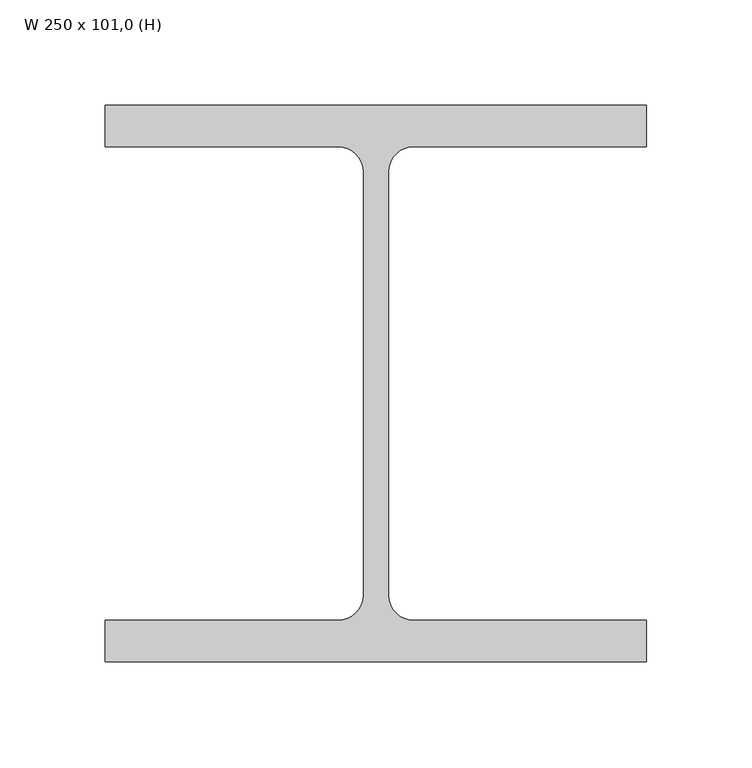
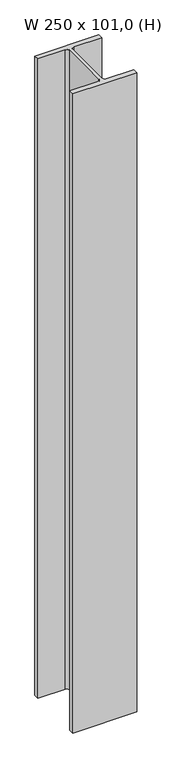
"""IFC4 building model written with IfcOpenShell, lengths in millimetres: column geometry, Pilar de Aço - H : W 250 x 101,0 (H)."""

from ifc_helpers import new_model, si_unit, point, frame_2d, origin, origin_with_axes, place, context, project, spatial, polyline, circle_curve, trimmed, segment, composite_curve, outline, extrude, source, transform, mapped, element, save


def w_250_x_101_0_h_e0a0315e(model_context):
    return source(origin(), model_context, "Body", "SweptSolid", [
        extrude(outline(composite_curve([segment(polyline([(128.5, 132.0), (128.5, 112.4), (17.85, 112.4)]), True, "CONTINUOUS"), segment(trimmed(circle_curve(frame_2d((17.85, 100.5)), 11.9), [point((17.85, 112.4))], [point((5.95, 100.5))], True, "CARTESIAN"), True, "CONTINUOUS"), segment(polyline([(5.95, 100.5), (5.95, -100.5)]), True, "CONTINUOUS"), segment(trimmed(circle_curve(frame_2d((17.85, -100.5)), 11.9), [point((5.95, -100.5))], [point((17.85, -112.4))], True, "CARTESIAN"), True, "CONTINUOUS"), segment(polyline([(17.85, -112.4), (128.5, -112.4), (128.5, -132.0), (-128.5, -132.0), (-128.5, -112.4), (-17.85, -112.4)]), True, "CONTINUOUS"), segment(trimmed(circle_curve(frame_2d((-17.85, -100.5)), 11.9), [point((-17.85, -112.4))], [point((-5.95, -100.5))], True, "CARTESIAN"), True, "CONTINUOUS"), segment(polyline([(-5.95, -100.5), (-5.95, 100.5)]), True, "CONTINUOUS"), segment(trimmed(circle_curve(frame_2d((-17.85, 100.5)), 11.9), [point((-5.95, 100.5))], [point((-17.85, 112.4))], True, "CARTESIAN"), True, "CONTINUOUS"), segment(polyline([(-17.85, 112.4), (-128.5, 112.4), (-128.5, 132.0), (128.5, 132.0)]), True, "CONTINUOUS")], self_intersect=False)), origin_with_axes(), (0.0, 0.0, 1.0), 2720.0),
    ])


if __name__ == "__main__":
    model = new_model("IFC4")
    model_context = context("Model", 3, world=origin())
    ifc_project = project(units=[si_unit("LENGTHUNIT", "METRE", prefix="MILLI")], contexts=[model_context])
    site = spatial("IfcSite", under=ifc_project)
    building = spatial("IfcBuilding", under=site)
    placement = place(None, origin())
    w_250_x_101_0_h_shape = w_250_x_101_0_h_e0a0315e(model_context)
    element("IfcColumn", 1, ObjectType="Pilar de Aço - H : W 250 x 101,0 (H)", at=placement, inside=building, context=model_context, shape_type="MappedRepresentation", body=[
        mapped(w_250_x_101_0_h_shape, transform((0.0, 0.0, 0.0), x_axis=(1.0, 0.0, 0.0), y_axis=(0.0, 1.0, 0.0), z_axis=(0.0, 0.0, 1.0))),
    ])
    save(model, "model.ifc")

# Revit data of these elements
# Type "Pilar de Aço - H : W 250 x 101,0 (H)"
#   SINAPI = ""
#   Área da seção = 128.7 m²
#   tw = 1.19 cm
#   tf = 1.96 cm
#   h = 22.48 cm
#   d' = 20.10 cm
#   d = 26.40 cm
#   bf = 25.70 cm
#   R = 1.19 cm
#   Massa Linear kg/m = 101
#   Aço = Metal - Aço 345MPa
#   Assembly Code = ""
# Materials
#   "Metal - Aço 345MPa": class "Metal", colour RGB 189 187 185, transparency 0, Cost = 0
